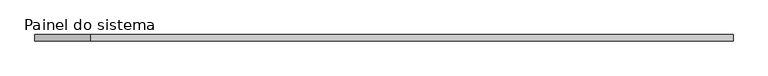
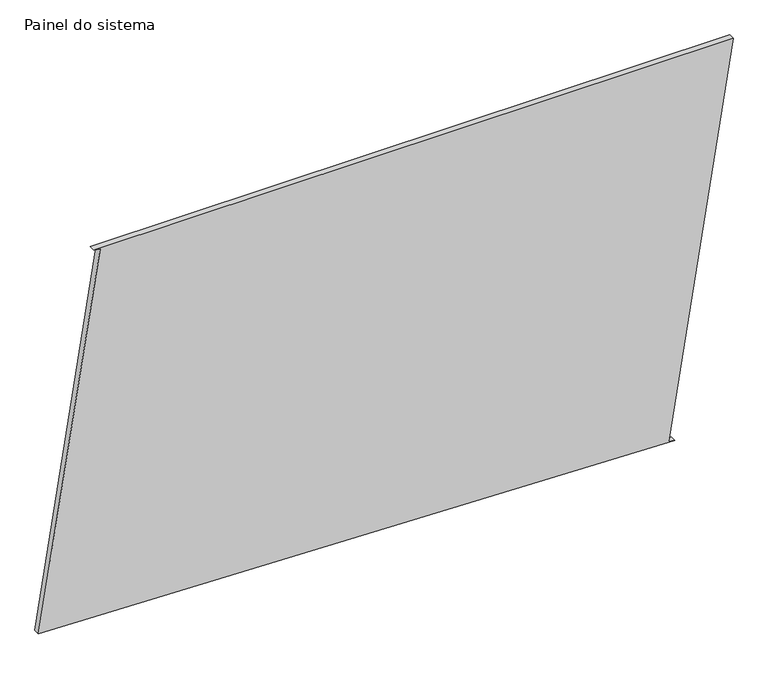
"""IFC4 building model written with IfcOpenShell, lengths in millimetres: plate geometry, Painel do sistema : Envidraçado."""

from ifc_helpers import new_model, si_unit, frame, origin, place, context, project, spatial, polyline, outline, extrude, source, transform, mapped, element, save


def painel_do_sistema_40bd1cf1(model_context):
    return source(origin(), model_context, "Body", "SweptSolid", [
        extrude(outline(polyline([(0.0, 1166.4304955), (3.9380954, 1141.7426158), (1634.3061082, 1401.8113125), (1634.3061082, -1178.0264128), (1630.3680129, -1153.338533), (72.6946874, -1401.8113125), (0.0, 1166.4304955)])), frame((0.0, 24.5, 0.0), z_axis=(0.0, 1.0, 0.0), x_axis=(0.0, 0.0, 1.0)), (0.0, 0.0, 1.0), 25.0),
    ])


if __name__ == "__main__":
    model = new_model("IFC4")
    model_context = context("Model", 3, world=origin())
    ifc_project = project(units=[si_unit("LENGTHUNIT", "METRE", prefix="MILLI")], contexts=[model_context])
    site = spatial("IfcSite", under=ifc_project)
    building = spatial("IfcBuilding", under=site)
    placement = place(None, origin())
    painel_do_sistema_shape = painel_do_sistema_40bd1cf1(model_context)
    element("IfcPlate", 1, ObjectType="Painel do sistema : Envidraçado", at=placement, inside=building, context=model_context, shape_type="MappedRepresentation", body=[
        mapped(painel_do_sistema_shape, transform((0.0, 0.0, 0.0), x_axis=(1.0, 0.0, 0.0), y_axis=(0.0, 1.0, 0.0), z_axis=(0.0, 0.0, 1.0))),
    ])
    save(model, "model.ifc")

# Revit data of these elements
# Type "Painel do sistema : Envidraçado"
#   Construction Type Id = "GSP4R"
#   Analytic Construction = "Vidraça única Pilkington 1/8 pol"
#   Visual Light Transmittance = 0.9
#   Solar Heat Gain Coefficient = 0.86
#   Heat Transfer Coefficient (U) = 6.7069 W/(m²·K)
# Element 1 (IfcPlate, "Painel do sistema : Envidraçado")
#   Materials on its faces: "Vidro"
# Materials
#   "Vidro": class "Vidro", colour RGB 0 128 192, transparency 0.9, Description = "Vidro de sílica", Cost = 0
